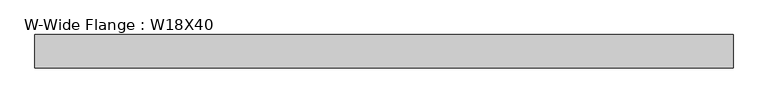
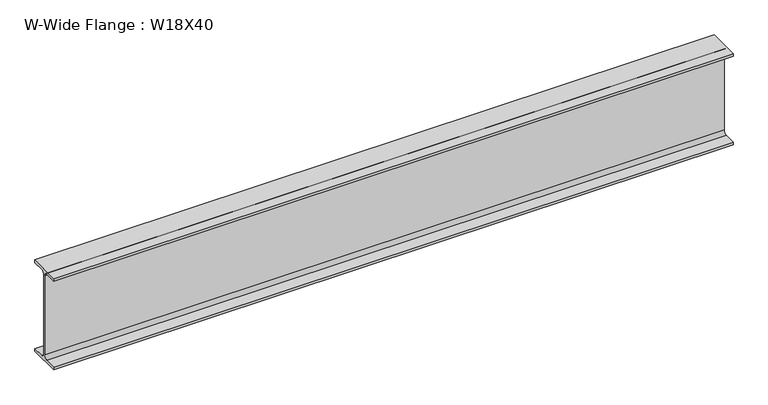
"""IFC4 building model written with IfcOpenShell, lengths in millimetres: beam geometry, W-Wide Flange : W18X40."""

from ifc_helpers import new_model, si_unit, point, frame, frame_2d, origin, place, context, project, spatial, polyline, circle_curve, trimmed, segment, composite_curve, outline, extrude, source, transform, mapped, element, save


def w_wide_flange_w18x40_572ee2a1(model_context):
    return source(origin(), model_context, "Body", "SweptSolid", [
        extrude(outline(composite_curve([segment(polyline([(76.454, -213.995), (76.454, -227.33), (-76.454, -227.33), (-76.454, -213.995), (-20.828, -213.995)]), True, "CONTINUOUS"), segment(trimmed(circle_curve(frame_2d((-20.828, -197.1675)), 16.8275), [point((-20.828, -213.995))], [point((-4.0005, -197.1675))], True, "CARTESIAN"), True, "CONTINUOUS"), segment(polyline([(-4.0005, -197.1675), (-4.0005, 197.1675)]), True, "CONTINUOUS"), segment(trimmed(circle_curve(frame_2d((-20.828, 197.1675)), 16.8275), [point((-4.0005, 197.1675))], [point((-20.828, 213.995))], True, "CARTESIAN"), True, "CONTINUOUS"), segment(polyline([(-20.828, 213.995), (-76.454, 213.995), (-76.454, 227.33), (76.454, 227.33), (76.454, 213.995), (20.828, 213.995)]), True, "CONTINUOUS"), segment(trimmed(circle_curve(frame_2d((20.828, 197.1675)), 16.8275), [point((20.828, 213.995))], [point((4.0005, 197.1675))], True, "CARTESIAN"), True, "CONTINUOUS"), segment(polyline([(4.0005, 197.1675), (4.0005, -197.1675)]), True, "CONTINUOUS"), segment(trimmed(circle_curve(frame_2d((20.828, -197.1675)), 16.8275), [point((4.0005, -197.1675))], [point((20.828, -213.995))], True, "CARTESIAN"), True, "CONTINUOUS"), segment(polyline([(20.828, -213.995), (76.454, -213.995)]), True, "CONTINUOUS")], self_intersect=False)), frame((-1562.1, 0.0, 0.0), z_axis=(1.0, 0.0, 0.0), x_axis=(0.0, 1.0, 0.0)), (0.0, 0.0, 1.0), 3200.3999994),
    ])


if __name__ == "__main__":
    model = new_model("IFC4")
    model_context = context("Model", 3, world=origin())
    ifc_project = project(units=[si_unit("LENGTHUNIT", "METRE", prefix="MILLI")], contexts=[model_context])
    site = spatial("IfcSite", under=ifc_project)
    building = spatial("IfcBuilding", under=site)
    placement = place(None, origin())
    w_wide_flange_w18x40_shape = w_wide_flange_w18x40_572ee2a1(model_context)
    element("IfcBeam", 1, ObjectType="W-Wide Flange : W18X40", at=placement, inside=building, context=model_context, shape_type="MappedRepresentation", body=[
        mapped(w_wide_flange_w18x40_shape, transform((0.0, 0.0, 0.0), x_axis=(1.0, 0.0, 0.0), y_axis=(0.0, 1.0, 0.0), z_axis=(0.0, 0.0, 1.0))),
    ])
    save(model, "model.ifc")

# Revit data of these elements
# Type "W-Wide Flange : W18X40"
#   Assembly Code = "B10"
#   W = 40
#   Length [instance default] = 5' - 0"
#   bf = 0' - 6.02"
#   d = 1' - 5.9"
#   k = 0' - 1 3/16"
#   k2 = 0' - 0.6625"
#   tf = 0' - 0.525"
#   tw = 0' - 0.315"
#   A = 0.0819444 SF
#   Structural Material [instance default] = Steel ASTM A992
# Element 1 (IfcBeam, "W-Wide Flange : W18X40")
#   Materials on its faces: "Steel ASTM A992"
# Materials
#   "Steel ASTM A992": class "Metal", colour RGB 199 199 199, transparency 0, Description = "Structural steel 50ksi", Cost = 0
